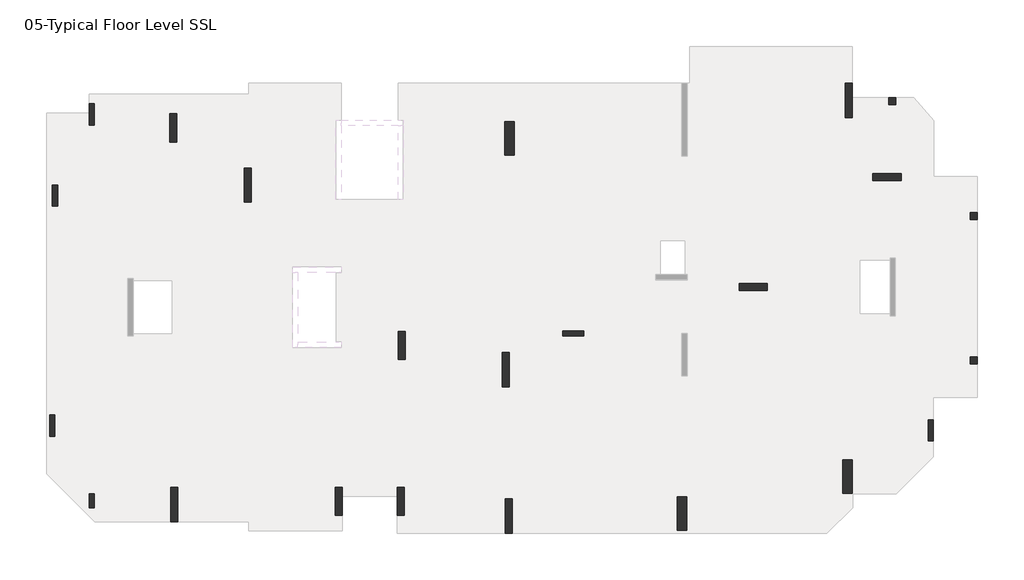
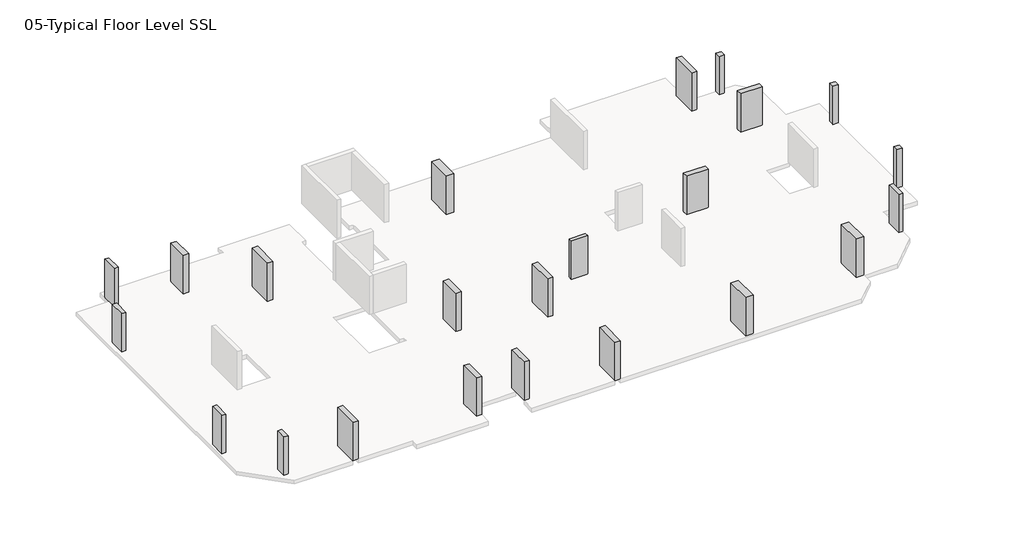
# One storey, part 2 of 2: 23 columns.
"""IFC4 building model written with IfcOpenShell, lengths in millimetres."""

from ifc_helpers import new_model, si_unit, origin, place, context, project, spatial, faceted_brep, element, save

model = new_model("IFC4")

# Units and contexts
model_context = context("Model", 3, world=origin())
ifc_project = project(units=[si_unit("LENGTHUNIT", "METRE", prefix="MILLI")], contexts=[model_context])

# Site, building, storey
site = spatial("IfcSite", under=ifc_project)
building = spatial("IfcBuilding", under=site)
storey = spatial("IfcBuildingStorey", under=building, Name="05-Typical Floor Level SSL", Elevation=9000.0)

# Columns
placement = place(None, origin())
element("IfcColumn", 1, ObjectType="M_Concrete-Rectangular-Column : C-1 (400 x 400mm)", at=placement, inside=storey, context=model_context, shape_type="Brep", body=[
    faceted_brep([(52549.9999998, 16712.0, 9000.0), (52549.9999998, 16312.0, 9000.0), (52149.9999998, 16312.0, 9000.0), (52149.9999998, 16712.0, 9000.0), (52549.9999998, 16712.0, 12000.0), (52549.9999998, 16312.0, 12000.0), (52549.9999998, 16312.0, 11700.0), (52549.9999998, 16712.0, 11700.0), (52149.9999998, 16312.0, 12000.0), (52149.9999998, 16312.0, 11700.0), (52149.9999998, 16712.0, 12000.0), (52149.9999998, 16712.0, 11700.0)], [[[0, 1, 2, 3]], [[4, 5, 6, 1, 0, 7]], [[5, 8, 9, 2, 1, 6]], [[8, 10, 11, 3, 2, 9]], [[10, 4, 7, 0, 3, 11]], [[4, 10, 8, 5]]]),
])
element("IfcColumn", 2, ObjectType="M_Concrete-Rectangular-Column : C-1 (400 x 400mm)", at=placement, inside=storey, context=model_context, shape_type="Brep", body=[
    faceted_brep([(47898.6337868, 23252.0, 9000.0), (47898.6337868, 22852.0, 9000.0), (47498.6337868, 22852.0, 9000.0), (47498.6337868, 23252.0, 9000.0), (47898.6337868, 23252.0, 12000.0), (47898.6337868, 22852.0, 12000.0), (47898.6337868, 22852.0, 11700.0), (47498.6337868, 22852.0, 12000.0), (47498.6337868, 22852.0, 11700.0), (47498.6337868, 23252.0, 12000.0)], [[[0, 1, 2, 3]], [[4, 5, 6, 1, 0]], [[5, 7, 8, 2, 1, 6]], [[7, 9, 3, 2, 8]], [[9, 4, 0, 3]], [[4, 9, 7, 5]]]),
])
element("IfcColumn", 3, ObjectType="M_Concrete-Rectangular-Column : C-1 (400 x 400mm)", at=placement, inside=storey, context=model_context, shape_type="Brep", body=[
    faceted_brep([(52549.9999998, 8504.0039609, 9000.0), (52549.9999998, 8104.0039609, 9000.0), (52149.9999998, 8104.0039609, 9000.0), (52149.9999998, 8504.0039609, 9000.0), (52549.9999998, 8504.0039609, 12000.0), (52549.9999998, 8104.0039609, 12000.0), (52549.9999998, 8104.0039609, 11700.0), (52549.9999998, 8504.0039609, 11700.0), (52149.9999998, 8104.0039609, 12000.0), (52149.9999998, 8104.0039609, 11700.0), (52149.9999998, 8504.0039609, 12000.0), (52149.9999998, 8504.0039609, 11700.0)], [[[0, 1, 2, 3]], [[4, 5, 6, 1, 0, 7]], [[5, 8, 9, 2, 1, 6]], [[8, 10, 11, 3, 2, 9]], [[10, 4, 7, 0, 3, 11]], [[4, 10, 8, 5]]]),
])
element("IfcColumn", 4, ObjectType="M_Concrete-Rectangular-Column : C-2 (300 x 800mm)", at=placement, inside=storey, context=model_context, shape_type="Brep", body=[
    faceted_brep([(2352.0, 728.0, 9000.0), (2352.0, -72.0, 9000.0), (2052.0, -72.0, 9000.0), (2052.0, 728.0, 9000.0), (2352.0, 728.0, 12000.0), (2352.0, -72.0, 12000.0), (2352.0, -72.0, 11700.0), (2352.0, 728.0, 11700.0), (2052.0, -72.0, 12000.0), (2052.0, -72.0, 11700.0), (2052.0, 728.0, 12000.0), (2052.0, 728.0, 11700.0)], [[[0, 1, 2, 3]], [[4, 5, 6, 1, 0, 7]], [[5, 8, 9, 2, 1, 6]], [[8, 10, 11, 3, 2, 9]], [[10, 4, 7, 0, 3, 11]], [[4, 10, 8, 5]]]),
])
element("IfcColumn", 5, ObjectType="M_Concrete-Rectangular-Column : C-3(300 x 1200mm)", at=placement, inside=storey, context=model_context, shape_type="Brep", body=[
    faceted_brep([(2352.0, 22908.0000656, 9000.0), (2352.0, 21708.0000656, 9000.0), (2052.0, 21708.0000656, 9000.0), (2052.0, 22908.0000656, 9000.0), (2352.0, 22908.0000656, 12000.0), (2352.0, 21708.0000656, 12000.0), (2352.0, 21708.0000656, 11700.0), (2352.0, 22908.0000656, 11700.0), (2052.0, 21708.0000656, 12000.0), (2052.0, 21708.0000656, 11700.0), (2052.0, 22380.0004589, 12000.0), (2052.0, 22908.0000656, 12000.0), (2052.0, 22908.0000656, 11700.0)], [[[0, 1, 2, 3]], [[4, 5, 6, 1, 0, 7]], [[5, 8, 9, 2, 1, 6]], [[8, 10, 11, 12, 3, 2, 9]], [[11, 4, 7, 0, 3, 12]], [[4, 11, 10, 8, 5]]]),
])
element("IfcColumn", 6, ObjectType="M_Concrete-Rectangular-Column : C-3(300 x 1200mm)", at=placement, inside=storey, context=model_context, shape_type="Brep", body=[
    faceted_brep([(257.9999999, 18288.0, 9000.0), (257.9999999, 17088.0, 9000.0), (-42.0000001, 17088.0, 9000.0), (-42.0000001, 18288.0, 9000.0), (257.9999999, 18288.0, 12000.0), (257.9999999, 17088.0, 12000.0), (257.9999999, 17088.0, 11700.0), (257.9999999, 18288.0, 11700.0), (-42.0000001, 17088.0, 12000.0), (-42.0000001, 17088.0, 11700.0), (-42.0000001, 18288.0, 12000.0), (-42.0000001, 18288.0, 11700.0)], [[[0, 1, 2, 3]], [[4, 5, 6, 1, 0, 7]], [[5, 8, 9, 2, 1, 6]], [[8, 10, 11, 3, 2, 9]], [[10, 4, 7, 0, 3, 11]], [[4, 10, 8, 5]]]),
])
element("IfcColumn", 7, ObjectType="M_Concrete-Rectangular-Column : C-3(300 x 1200mm)", at=placement, inside=storey, context=model_context, shape_type="Brep", body=[
    faceted_brep([(108.001803, 5201.9999858, 9000.0), (108.001803, 4001.9999858, 9000.0), (-191.998197, 4001.9999858, 9000.0), (-191.998197, 5201.9999858, 9000.0), (108.001803, 5201.9999858, 12000.0), (108.001803, 4001.9999858, 12000.0), (108.001803, 4001.9999858, 11700.0), (108.001803, 5201.9999858, 11700.0), (-191.998197, 4001.9999858, 12000.0), (-191.998197, 4001.9999858, 11700.0), (-191.998197, 5201.9999858, 12000.0), (-191.998197, 5201.9999858, 11700.0)], [[[0, 1, 2, 3]], [[4, 5, 6, 1, 0, 7]], [[5, 8, 9, 2, 1, 6]], [[8, 10, 11, 3, 2, 9]], [[10, 4, 7, 0, 3, 11]], [[4, 10, 8, 5]]]),
])
element("IfcColumn", 8, ObjectType="M_Concrete-Rectangular-Column : C-3(300 x 1200mm)", at=placement, inside=storey, context=model_context, shape_type="Brep", body=[
    faceted_brep([(50046.0009271, 4931.9999929, 9000.0), (50046.0009271, 3731.9999929, 9000.0), (49746.0009271, 3731.9999929, 9000.0), (49746.0009271, 4931.9999929, 9000.0), (50046.0009271, 4931.9999929, 12000.0), (50046.0009271, 3731.9999929, 12000.0), (50046.0009271, 3731.9999929, 11700.0), (50046.0009271, 4931.9999929, 11700.0), (49746.0009271, 3731.9999929, 12000.0), (49746.0009271, 3731.9999929, 11700.0), (49746.0009271, 4931.9999929, 12000.0), (49746.0009271, 4931.9999929, 11700.0)], [[[0, 1, 2, 3]], [[4, 5, 6, 1, 0, 7]], [[5, 8, 9, 2, 1, 6]], [[8, 10, 11, 3, 2, 9]], [[10, 4, 7, 0, 3, 11]], [[4, 10, 8, 5]]]),
])
element("IfcColumn", 9, ObjectType="M_Concrete-Rectangular-Column : C-3(300 x 1200mm)", at=placement, inside=storey, context=model_context, shape_type="Brep", body=[
    faceted_brep([(28975.9999998, 9996.0000019, 9000.0), (30175.9999998, 9996.0000019, 9000.0), (30175.9999998, 9696.0000019, 9000.0), (28975.9999998, 9696.0000019, 9000.0), (28975.9999998, 9996.0000019, 12000.0), (30175.9999998, 9996.0000019, 12000.0), (30175.9999998, 9996.0000019, 11700.0), (28975.9999998, 9996.0000019, 11700.0), (30175.9999998, 9696.0000019, 12000.0), (30175.9999998, 9696.0000019, 11700.0), (28975.9999998, 9696.0000019, 12000.0), (28975.9999998, 9696.0000019, 11700.0)], [[[0, 1, 2, 3]], [[4, 5, 6, 1, 0, 7]], [[5, 8, 9, 2, 1, 6]], [[8, 10, 11, 3, 2, 9]], [[10, 4, 7, 0, 3, 11]], [[4, 10, 8, 5]]]),
])
element("IfcColumn", 10, ObjectType="M_Concrete-Rectangular-Column : C-4 (400 x 1600mm)", at=placement, inside=storey, context=model_context, shape_type="Brep", body=[
    faceted_brep([(7021.9999999, 22340.0000078, 9000.0), (7021.9999999, 20740.0000078, 9000.0), (6621.9999999, 20740.0000078, 9000.0), (6621.9999999, 22340.0000078, 9000.0), (7021.9999999, 22340.0000078, 12000.0), (7021.9999999, 20740.0000078, 12000.0), (7021.9999999, 20740.0000078, 11700.0), (7021.9999999, 22340.0000078, 11700.0), (6621.9999999, 20740.0000078, 12000.0), (6621.9999999, 20740.0000078, 11700.0), (6621.9999999, 22340.0000078, 12000.0), (6621.9999999, 22340.0000078, 11700.0)], [[[0, 1, 2, 3]], [[4, 5, 6, 1, 0, 7]], [[5, 8, 9, 2, 1, 6]], [[8, 10, 11, 3, 2, 9]], [[10, 4, 7, 0, 3, 11]], [[4, 10, 8, 5]]]),
])
element("IfcColumn", 11, ObjectType="M_Concrete-Rectangular-Column : C-4 (400 x 1600mm)", at=placement, inside=storey, context=model_context, shape_type="Brep", body=[
    faceted_brep([(19969.9997488, 1087.9955348, 9000.0), (19969.9997488, -512.0044652, 9000.0), (19569.9997488, -512.0044652, 9000.0), (19569.9997488, 1087.9955348, 9000.0), (19969.9997488, 1087.9955348, 12000.0), (19969.9997488, -512.0044652, 12000.0), (19969.9997488, -512.0044652, 11700.0), (19969.9997488, 1087.9955348, 11700.0), (19569.9997488, -512.0044652, 12000.0), (19569.9997488, -512.0044652, 11700.0), (19569.9997488, 564.000519, 12000.0), (19569.9997488, 1087.9955348, 12000.0), (19569.9997488, 1087.9955348, 11700.0)], [[[0, 1, 2, 3]], [[4, 5, 6, 1, 0, 7]], [[5, 8, 9, 2, 1, 6]], [[8, 10, 11, 12, 3, 2, 9]], [[11, 4, 7, 0, 3, 12]], [[4, 11, 10, 8, 5]]]),
])
element("IfcColumn", 12, ObjectType="M_Concrete-Rectangular-Column : C-4 (400 x 1600mm)", at=placement, inside=storey, context=model_context, shape_type="Brep", body=[
    faceted_brep([(46605.9993605, 18950.0, 9000.0), (48205.9993605, 18950.0, 9000.0), (48205.9993605, 18550.0, 9000.0), (46605.9993605, 18550.0, 9000.0), (46605.9993605, 18950.0, 12000.0), (48205.9993605, 18950.0, 12000.0), (48205.9993605, 18950.0, 11700.0), (46605.9993605, 18950.0, 11700.0), (48205.9993605, 18550.0, 12000.0), (48205.9993605, 18550.0, 11700.0), (46605.9993605, 18550.0, 12000.0), (46605.9993605, 18550.0, 11700.0)], [[[0, 1, 2, 3]], [[4, 5, 6, 1, 0, 7]], [[5, 8, 9, 2, 1, 6]], [[8, 10, 11, 3, 2, 9]], [[10, 4, 7, 0, 3, 11]], [[4, 10, 8, 5]]]),
])
element("IfcColumn", 13, ObjectType="M_Concrete-Rectangular-Column : C-5 (400 x 1600mm)", at=placement, inside=storey, context=model_context, shape_type="Brep", body=[
    faceted_brep([(20030.000009, 9955.9999979, 9000.0), (20030.000009, 8355.9999979, 9000.0), (19630.000009, 8355.9999979, 9000.0), (19630.000009, 9955.9999979, 9000.0), (20030.000009, 9955.9999979, 12000.0), (20030.000009, 8355.9999979, 12000.0), (20030.000009, 8355.9999979, 11700.0), (20030.000009, 9955.9999979, 11700.0), (19630.000009, 8355.9999979, 12000.0), (19630.000009, 8355.9999979, 11700.0), (19630.000009, 9955.9999979, 12000.0), (19630.000009, 9955.9999979, 11700.0)], [[[0, 1, 2, 3]], [[4, 5, 6, 1, 0, 7]], [[5, 8, 9, 2, 1, 6]], [[8, 10, 11, 3, 2, 9]], [[10, 4, 7, 0, 3, 11]], [[4, 10, 8, 5]]]),
])
element("IfcColumn", 14, ObjectType="M_Concrete-Rectangular-Column : C-5 (400 x 1600mm)", at=placement, inside=storey, context=model_context, shape_type="Brep", body=[
    faceted_brep([(16429.9999981, 1088.0, 9000.0), (16429.9999981, -512.0, 9000.0), (16029.9999981, -512.0, 9000.0), (16029.9999981, 1088.0, 9000.0), (16429.9999981, 1088.0, 12000.0), (16429.9999981, 564.000519, 12000.0), (16429.9999981, -512.0, 12000.0), (16429.9999981, -512.0, 11700.0), (16429.9999981, 1088.0, 11700.0), (16029.9999981, -512.0, 12000.0), (16029.9999981, -512.0, 11700.0), (16029.9999981, 1088.0, 12000.0), (16029.9999981, 1088.0, 11700.0)], [[[0, 1, 2, 3]], [[4, 5, 6, 7, 1, 0, 8]], [[6, 9, 10, 2, 1, 7]], [[9, 11, 12, 3, 2, 10]], [[11, 4, 8, 0, 3, 12]], [[4, 11, 9, 6, 5]]]),
])
element("IfcColumn", 15, ObjectType="M_Concrete-Rectangular-Column : C-5 (400 x 1600mm)", at=placement, inside=storey, context=model_context, shape_type="Brep", body=[
    faceted_brep([(38998.0014887, 12692.0079212, 9000.0), (40598.0014887, 12692.0079212, 9000.0), (40598.0014887, 12292.0079212, 9000.0), (38998.0014887, 12292.0079212, 9000.0), (38998.0014887, 12692.0079212, 12000.0), (40598.0014887, 12692.0079212, 12000.0), (40598.0014887, 12692.0079212, 11700.0), (38998.0014887, 12692.0079212, 11700.0), (40598.0014887, 12292.0079212, 12000.0), (40598.0014887, 12292.0079212, 11700.0), (38998.0014887, 12292.0079212, 12000.0), (38998.0014887, 12292.0079212, 11700.0)], [[[0, 1, 2, 3]], [[4, 5, 6, 1, 0, 7]], [[5, 8, 9, 2, 1, 6]], [[8, 10, 11, 3, 2, 9]], [[10, 4, 7, 0, 3, 11]], [[4, 10, 8, 5]]]),
])
element("IfcColumn", 16, ObjectType="M_Concrete-Rectangular-Column : C-6 (400 x 1950mm)", at=placement, inside=storey, context=model_context, shape_type="Brep", body=[
    faceted_brep([(11270.0000427, 19262.9999996, 9000.0), (11270.0000427, 17312.9999996, 9000.0), (10870.0000427, 17312.9999996, 9000.0), (10870.0000427, 19262.9999996, 9000.0), (11270.0000427, 19262.9999996, 12000.0), (11270.0000427, 17312.9999996, 12000.0), (11270.0000427, 17312.9999996, 11700.0), (11270.0000427, 19262.9999996, 11700.0), (10870.0000427, 17312.9999996, 12000.0), (10870.0000427, 17312.9999996, 11700.0), (10870.0000427, 19262.9999996, 12000.0), (10870.0000427, 19262.9999996, 11700.0)], [[[0, 1, 2, 3]], [[4, 5, 6, 1, 0, 7]], [[5, 8, 9, 2, 1, 6]], [[8, 10, 11, 3, 2, 9]], [[10, 4, 7, 0, 3, 11]], [[4, 10, 8, 5]]]),
])
element("IfcColumn", 17, ObjectType="M_Concrete-Rectangular-Column : C-6 (400 x 1950mm)", at=placement, inside=storey, context=model_context, shape_type="Brep", body=[
    faceted_brep([(7082.0000416, 1083.0000153, 9000.0), (7082.0000416, -866.9999847, 9000.0), (6682.0000416, -866.9999847, 9000.0), (6682.0000416, 1083.0000153, 9000.0), (7082.0000416, 1083.0000153, 12000.0), (7082.0000416, -866.9999847, 12000.0), (7082.0000416, -866.9999847, 11700.0), (7082.0000416, 1083.0000153, 11700.0), (6682.0000416, -866.9999847, 12000.0), (6682.0000416, -866.9999847, 11700.0), (6682.0000416, 1083.0000153, 12000.0), (6682.0000416, 1083.0000153, 11700.0)], [[[0, 1, 2, 3]], [[4, 5, 6, 1, 0, 7]], [[5, 8, 9, 2, 1, 6]], [[8, 10, 11, 3, 2, 9]], [[10, 4, 7, 0, 3, 11]], [[4, 10, 8, 5]]]),
])
element("IfcColumn", 18, ObjectType="M_Concrete-Rectangular-Column : C-6 (400 x 1950mm)", at=placement, inside=storey, context=model_context, shape_type="Brep", body=[
    faceted_brep([(26113.9999998, 422.995535, 9000.0), (26113.9999998, -1527.004465, 9000.0), (25713.9999998, -1527.004465, 9000.0), (25713.9999998, 422.995535, 9000.0), (26113.9999998, 422.995535, 12000.0), (26113.9999998, -1527.004465, 12000.0), (26113.9999998, -1527.004465, 11700.0), (26113.9999998, 422.995535, 11700.0), (25713.9999998, -1527.004465, 12000.0), (25713.9999998, -1527.004465, 11700.0), (25713.9999998, 422.995535, 12000.0), (25713.9999998, 422.995535, 11700.0)], [[[0, 1, 2, 3]], [[4, 5, 6, 1, 0, 7]], [[5, 8, 9, 2, 1, 6]], [[8, 10, 11, 3, 2, 9]], [[10, 4, 7, 0, 3, 11]], [[4, 10, 8, 5]]]),
])
element("IfcColumn", 19, ObjectType="M_Concrete-Rectangular-Column : C-6 (400 x 1950mm)", at=placement, inside=storey, context=model_context, shape_type="Brep", body=[
    faceted_brep([(45446.0007483, 24087.0, 9000.0), (45446.0007483, 22137.0, 9000.0), (45046.0007483, 22137.0, 9000.0), (45046.0007483, 24087.0, 9000.0), (45446.0007483, 24087.0, 12000.0), (45446.0007483, 23252.0000315, 12000.0), (45446.0007483, 22137.0, 12000.0), (45446.0007483, 22137.0, 11700.0), (45446.0007483, 24087.0, 11700.0), (45046.0007483, 22137.0, 12000.0), (45046.0007483, 22137.0, 11700.0), (45046.0007483, 24087.0, 12000.0), (45046.0007483, 24087.0, 11700.0)], [[[0, 1, 2, 3]], [[4, 5, 6, 7, 1, 0, 8]], [[6, 9, 10, 2, 1, 7]], [[9, 11, 12, 3, 2, 10]], [[11, 4, 8, 0, 3, 12]], [[4, 11, 9, 6, 5]]]),
])
element("IfcColumn", 20, ObjectType="M_Concrete-Rectangular-Column : C-6 (400 x 1950mm)", at=placement, inside=storey, context=model_context, shape_type="Brep", body=[
    faceted_brep([(25934.0000455, 8751.0001824, 9000.0), (25934.0000455, 6801.0001824, 9000.0), (25534.0000455, 6801.0001824, 9000.0), (25534.0000455, 8751.0001824, 9000.0), (25934.0000455, 8751.0001824, 12000.0), (25934.0000455, 6801.0001824, 12000.0), (25934.0000455, 6801.0001824, 11700.0), (25934.0000455, 8751.0001824, 11700.0), (25534.0000455, 6801.0001824, 12000.0), (25534.0000455, 6801.0001824, 11700.0), (25534.0000455, 8751.0001824, 12000.0), (25534.0000455, 8751.0001824, 11700.0)], [[[0, 1, 2, 3]], [[4, 5, 6, 1, 0, 7]], [[5, 8, 9, 2, 1, 6]], [[8, 10, 11, 3, 2, 9]], [[10, 4, 7, 0, 3, 11]], [[4, 10, 8, 5]]]),
])
element("IfcColumn", 21, ObjectType="M_Concrete-Rectangular-Column : C-7 (550 x 1900mm)", at=placement, inside=storey, context=model_context, shape_type="Brep", body=[
    faceted_brep([(36035.9999998, 548.0007983, 9000.0), (36035.9999998, -1351.9992017, 9000.0), (35485.9999998, -1351.9992017, 9000.0), (35485.9999998, 548.0007983, 9000.0), (36035.9999998, 548.0007983, 12000.0), (36035.9999998, -1351.9992017, 12000.0), (36035.9999998, -1351.9992017, 11700.0), (36035.9999998, 548.0007983, 11700.0), (35485.9999998, -1351.9992017, 12000.0), (35485.9999998, -1351.9992017, 11700.0), (35485.9999998, 548.0007983, 12000.0), (35485.9999998, 548.0007983, 11700.0)], [[[0, 1, 2, 3]], [[4, 5, 6, 1, 0, 7]], [[5, 8, 9, 2, 1, 6]], [[8, 10, 11, 3, 2, 9]], [[10, 4, 7, 0, 3, 11]], [[4, 10, 8, 5]]]),
])
element("IfcColumn", 22, ObjectType="M_Concrete-Rectangular-Column : C-7 (550 x 1900mm)", at=placement, inside=storey, context=model_context, shape_type="Brep", body=[
    faceted_brep([(45443.9999998, 2648.0, 9000.0), (45443.9999998, 748.0, 9000.0), (44893.9999998, 748.0, 9000.0), (44893.9999998, 2648.0, 9000.0), (45443.9999998, 2648.0, 12000.0), (45443.9999998, 748.0, 12000.0), (45443.9999998, 748.0, 11700.0), (45443.9999998, 2648.0, 11700.0), (44893.9999998, 748.0, 12000.0), (44893.9999998, 748.0, 11700.0), (44893.9999998, 2648.0, 12000.0), (44893.9999998, 2648.0, 11700.0)], [[[0, 1, 2, 3]], [[4, 5, 6, 1, 0, 7]], [[5, 8, 9, 2, 1, 6]], [[8, 10, 11, 3, 2, 9]], [[10, 4, 7, 0, 3, 11]], [[4, 10, 8, 5]]]),
])
element("IfcColumn", 23, ObjectType="M_Concrete-Rectangular-Column : C-7 (550 x 1900mm)", at=placement, inside=storey, context=model_context, shape_type="Brep", body=[
    faceted_brep([(26218.9999998, 21900.0, 9000.0), (26218.9999998, 20000.0, 9000.0), (25668.9999998, 20000.0, 9000.0), (25668.9999998, 21900.0, 9000.0), (26218.9999998, 21900.0, 12000.0), (26218.9999998, 20000.0, 12000.0), (26218.9999998, 20000.0, 11700.0), (26218.9999998, 21900.0, 11700.0), (25668.9999998, 20000.0, 12000.0), (25668.9999998, 20000.0, 11700.0), (25668.9999998, 21900.0, 12000.0), (25668.9999998, 21900.0, 11700.0)], [[[0, 1, 2, 3]], [[4, 5, 6, 1, 0, 7]], [[5, 8, 9, 2, 1, 6]], [[8, 10, 11, 3, 2, 9]], [[10, 4, 7, 0, 3, 11]], [[4, 10, 8, 5]]]),
])

save(model, "model.ifc")

# Revit data of these elements
# Type "M_Concrete-Rectangular-Column : C-1 (400 x 400mm)"
#   Type Mark = "C01"
#   b = 400 mm
#   h = 400 mm
#   Structural Material [instance default] = Concrete, Cast-in-Place gray
# Type "M_Concrete-Rectangular-Column : C-2 (300 x 800mm)"
#   Type Mark = "C02"
#   b = 300 mm
#   h = 800 mm
#   Structural Material [instance default] = Concrete, Cast-in-Place gray
# Type "M_Concrete-Rectangular-Column : C-3(300 x 1200mm)"
#   Type Mark = "C03"
#   b = 300 mm
#   h = 1200 mm
#   Structural Material [instance default] = Concrete, Cast-in-Place gray
# Type "M_Concrete-Rectangular-Column : C-4 (400 x 1600mm)"
#   Type Mark = "C04"
#   b = 400 mm
#   h = 1600 mm
#   Structural Material [instance default] = Concrete, Cast-in-Place gray
# Type "M_Concrete-Rectangular-Column : C-5 (400 x 1600mm)"
#   Type Mark = "C05"
#   b = 400 mm
#   h = 1600 mm
#   Structural Material [instance default] = Concrete, Cast-in-Place gray
# Type "M_Concrete-Rectangular-Column : C-6 (400 x 1950mm)"
#   Type Mark = "C06"
#   b = 400 mm
#   h = 1950 mm
#   Structural Material [instance default] = Concrete, Cast-in-Place gray
# Type "M_Concrete-Rectangular-Column : C-7 (550 x 1900mm)"
#   Type Mark = "C07"
#   b = 550 mm
#   h = 1900 mm
#   Structural Material [instance default] = Concrete, Cast-in-Place gray
# Elements 1, 2, 3 (IfcColumn, "M_Concrete-Rectangular-Column : C-1 (400 x 400mm)")
#   Structural Material = Concrete-RC
#   Phase Created = New Construction
#   Materials on its faces: "Concrete-RC"
# Element 4 (IfcColumn, "M_Concrete-Rectangular-Column : C-2 (300 x 800mm)")
#   Structural Material = Concrete-RC
#   Phase Created = New Construction
#   Materials on its faces: "Concrete-RC"
# Elements 5, 6, 7, 8, 9 (IfcColumn, "M_Concrete-Rectangular-Column : C-3(300 x 1200mm)")
#   Structural Material = Concrete-RC
#   Phase Created = New Construction
#   Materials on its faces: "Concrete-RC"
# Elements 10, 11, 12 (IfcColumn, "M_Concrete-Rectangular-Column : C-4 (400 x 1600mm)")
#   Structural Material = Concrete-RC
#   Phase Created = New Construction
#   Materials on its faces: "Concrete-RC"
# Elements 13, 14, 15 (IfcColumn, "M_Concrete-Rectangular-Column : C-5 (400 x 1600mm)")
#   Structural Material = Concrete-RC
#   Phase Created = New Construction
#   Materials on its faces: "Concrete-RC"
# Elements 16, 17, 18, 19, 20 (IfcColumn, "M_Concrete-Rectangular-Column : C-6 (400 x 1950mm)")
#   Structural Material = Concrete-RC
#   Phase Created = New Construction
#   Materials on its faces: "Concrete-RC"
# Elements 21, 22, 23 (IfcColumn, "M_Concrete-Rectangular-Column : C-7 (550 x 1900mm)")
#   Structural Material = Concrete-RC
#   Phase Created = New Construction
#   Materials on its faces: "Concrete-RC"
# Materials
#   "Concrete, Cast-in-Place gray": class "Concrete", colour RGB 192 192 192, transparency 0, Description = "Cast-in-place concrete", Cost = 0
#   "Concrete-RC": class "Concrete", colour RGB 128 128 128, transparency 0, Description = "High strength concrete", Cost = 0
